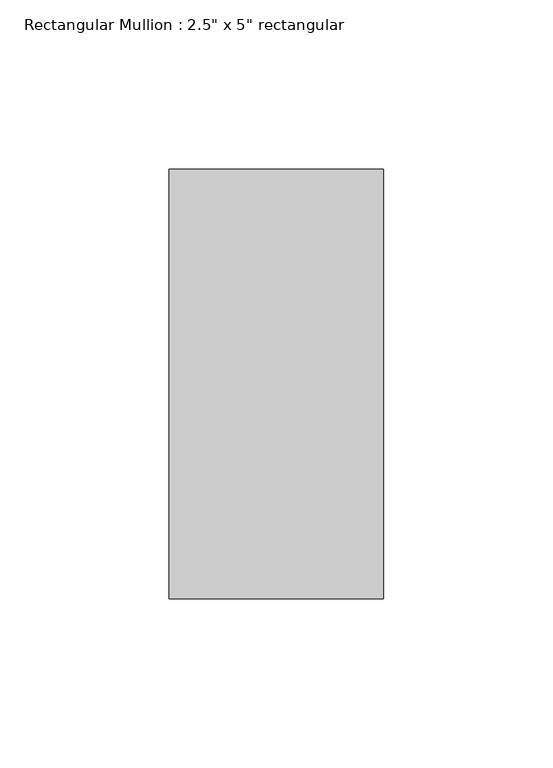
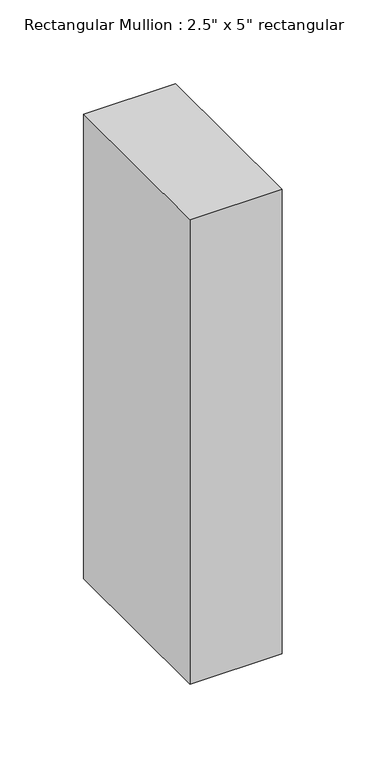
"""IFC4 building model written with IfcOpenShell, lengths in millimetres: member geometry."""

from ifc_helpers import new_model, si_unit, frame, origin, place, context, project, spatial, polyline, outline, extrude, source, transform, mapped, element, save


def member_6da2ef55(model_context):
    return source(origin(), model_context, "Body", "SweptSolid", [
        extrude(outline(polyline([(31.75, 63.5), (31.75, -63.5), (-31.75, -63.5), (-31.75, 63.5), (31.75, 63.5)])), frame((0.0, 0.0, -338.3578591), z_axis=(0.0, 0.0, 1.0), x_axis=(1.0, 0.0, 0.0)), (0.0, 0.0, 1.0), 338.3578591),
    ])


if __name__ == "__main__":
    model = new_model("IFC4")
    model_context = context("Model", 3, world=origin())
    ifc_project = project(units=[si_unit("LENGTHUNIT", "METRE", prefix="MILLI")], contexts=[model_context])
    site = spatial("IfcSite", under=ifc_project)
    building = spatial("IfcBuilding", under=site)
    placement = place(None, origin())
    member_shape = member_6da2ef55(model_context)
    element("IfcMember", 1, ObjectType="Rectangular Mullion : 2.5\" x 5\" rectangular", at=placement, inside=building, context=model_context, shape_type="MappedRepresentation", body=[
        mapped(member_shape, transform((0.0, 0.0, 0.0), x_axis=(1.0, 0.0, 0.0), y_axis=(0.0, 1.0, 0.0), z_axis=(0.0, 0.0, 1.0))),
    ])
    save(model, "model.ifc")

# Revit data of these elements
# Type "Rectangular Mullion : 2.5\" x 5\" rectangular"
#   built-in parameter 1007304 = 0.416667 (stored number, unit not read)
#   built-in parameter 1007301 = 0.104167 (stored number, unit not read)
#   built-in parameter 1007300 = 0.104167 (stored number, unit not read)
# Element 1 (IfcMember, "Rectangular Mullion : 2.5\" x 5\" rectangular")
#   Materials on its faces: "Metal - Aluminum 2"
# Materials
#   "Metal - Aluminum 2": class "Metal", colour RGB 189 187 185, transparency 0
